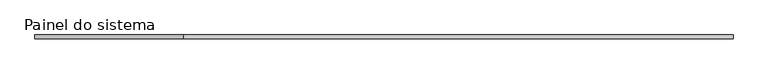
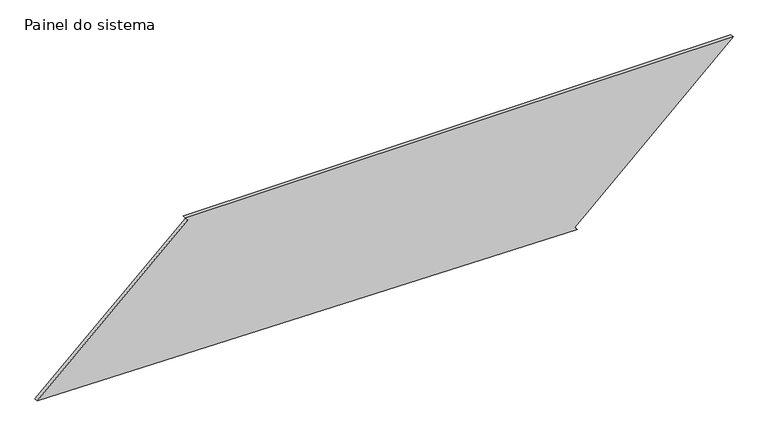
"""IFC4 building model written with IfcOpenShell, lengths in millimetres: plate geometry, Painel do sistema : Envidraçado."""

from ifc_helpers import new_model, si_unit, frame, origin, place, context, project, spatial, polyline, outline, extrude, source, transform, mapped, element, save


def painel_do_sistema_f3bd26b0(model_context):
    return source(origin(), model_context, "Body", "SweptSolid", [
        extrude(outline(polyline([(0.0, 1316.5486047), (18.3764951, 1299.5985479), (1021.2720041, 2386.8930988), (1021.2720041, -1370.6591069), (1002.895509, -1353.70905), (49.9102838, -2386.8930988), (0.0, 1316.5486047)])), frame((0.0, 24.5, 0.0), z_axis=(0.0, 1.0, 0.0), x_axis=(0.0, 0.0, 1.0)), (0.0, 0.0, 1.0), 25.0),
    ])


if __name__ == "__main__":
    model = new_model("IFC4")
    model_context = context("Model", 3, world=origin())
    ifc_project = project(units=[si_unit("LENGTHUNIT", "METRE", prefix="MILLI")], contexts=[model_context])
    site = spatial("IfcSite", under=ifc_project)
    building = spatial("IfcBuilding", under=site)
    placement = place(None, origin())
    painel_do_sistema_shape = painel_do_sistema_f3bd26b0(model_context)
    element("IfcPlate", 1, ObjectType="Painel do sistema : Envidraçado", at=placement, inside=building, context=model_context, shape_type="MappedRepresentation", body=[
        mapped(painel_do_sistema_shape, transform((0.0, 0.0, 0.0), x_axis=(1.0, 0.0, 0.0), y_axis=(0.0, 1.0, 0.0), z_axis=(0.0, 0.0, 1.0))),
    ])
    save(model, "model.ifc")

# Revit data of these elements
# Type "Painel do sistema : Envidraçado"
#   Construction Type Id = "GSP4R"
#   Analytic Construction = "Vidraça única Pilkington 1/8 pol"
#   Visual Light Transmittance = 0.9
#   Solar Heat Gain Coefficient = 0.86
#   Heat Transfer Coefficient (U) = 6.7069 W/(m²·K)
# Element 1 (IfcPlate, "Painel do sistema : Envidraçado")
#   Materials on its faces: "Vidro"
# Materials
#   "Vidro": class "Vidro", colour RGB 0 128 192, transparency 0.9, Description = "Vidro de sílica", Cost = 0
